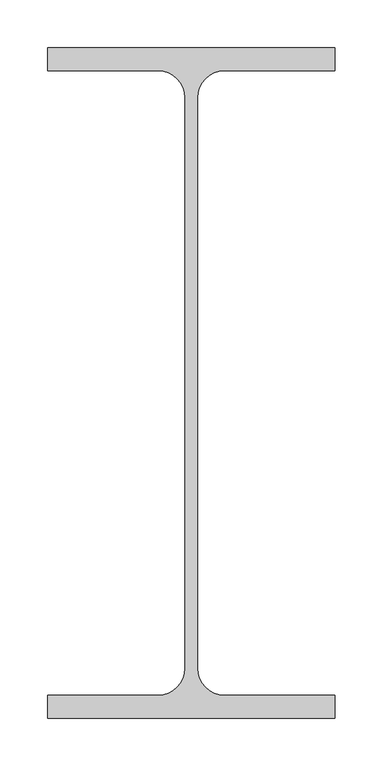
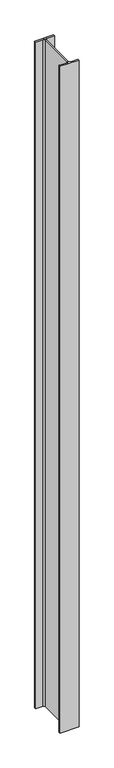
"""IFC4 building model written with IfcOpenShell, lengths in millimetres: column geometry, 0912_Steel Column_H_KSD3502 : H_SC_ASC_H-700x300x13x24."""

import ifcopenshell
import ifcopenshell.guid

model = None  # the IFC model being written
_history = None  # IfcOwnerHistory: only IFC2X3 demands one
_inside = {}  # id of a spatial element -> (the spatial element, [elements in it])
_under = {}  # id of a project, library or spatial element -> (it, [spatial elements below it])
_declared = {}  # id of a project -> (the project, [libraries it declares])
_typed = {}  # id of a type object -> (the type object, [elements of that type])
_made_of = {}  # id of a material, layer set ... -> (it, [elements and type objects made of it])


def new_model(schema):
    """Start an empty IFC model of exactly this schema.

    Asked for "IFC4X3", IfcOpenShell would pick the latest addendum, in which some entities
    have other attributes; the version numbers below select the first issue.
    IFC2X3 requires an IfcOwnerHistory on every rooted entity: one is made here for all.
    """
    global model, _history
    if schema == "IFC4X3":
        model = ifcopenshell.file(schema_version=(4, 3, 0, 0))
    else:
        model = ifcopenshell.file(schema=schema)
    _inside.clear()
    _under.clear()
    _declared.clear()
    _typed.clear()
    _made_of.clear()
    _history = None
    if model.schema == "IFC2X3":
        org = make("IfcOrganization", Name="unknown")
        user = make(
            "IfcPersonAndOrganization",
            ThePerson=make("IfcPerson", FamilyName="unknown"),
            TheOrganization=org,
        )
        app = make(
            "IfcApplication",
            ApplicationDeveloper=org,
            Version="unknown",
            ApplicationFullName="unknown",
            ApplicationIdentifier="unknown",
        )
        _history = make(
            "IfcOwnerHistory",
            OwningUser=user,
            OwningApplication=app,
            ChangeAction="ADDED",
            CreationDate=0,
        )
    return model


def make(cls, **values):
    """One entity of the class cls with the attributes given. An attribute that is None is left unset."""
    return model.create_entity(
        cls, **{name: value for name, value in values.items() if value is not None}
    )


def rooted(cls, **values):
    """An entity with a GlobalId (a new one), such as an element, a storey or a relation."""
    return make(cls, GlobalId=ifcopenshell.guid.new(), OwnerHistory=_history, **values)


def si_unit(unit_type, name, prefix=None):
    """IfcSIUnit, for example si_unit("LENGTHUNIT", "METRE", prefix="MILLI")."""
    return make("IfcSIUnit", UnitType=unit_type, Prefix=prefix, Name=name)


def assignment(units):
    """IfcUnitAssignment: the units of a project."""
    return None if units is None else make("IfcUnitAssignment", Units=units)


def point(xyz):
    """IfcCartesianPoint."""
    return None if xyz is None else make("IfcCartesianPoint", Coordinates=xyz)


def direction(xyz):
    """IfcDirection."""
    return None if xyz is None else make("IfcDirection", DirectionRatios=xyz)


def frame(location, z_axis=None, x_axis=None):
    """IfcAxis2Placement3D, a coordinate frame: its origin and axes. An axis left out is left unset."""
    return make(
        "IfcAxis2Placement3D",
        Location=point(location),
        Axis=direction(z_axis),
        RefDirection=direction(x_axis),
    )


def frame_2d(location, x_axis=None):
    """IfcAxis2Placement2D, a coordinate frame in the plane: its origin and x axis."""
    return make(
        "IfcAxis2Placement2D", Location=point(location), RefDirection=direction(x_axis)
    )


def origin():
    """The frame at (0, 0, 0) with its axes left unset."""
    return frame((0.0, 0.0, 0.0))


def origin_with_axes():
    """The frame at (0, 0, 0) with the z axis (0, 0, 1) and the x axis (1, 0, 0) written out."""
    return frame((0.0, 0.0, 0.0), z_axis=(0.0, 0.0, 1.0), x_axis=(1.0, 0.0, 0.0))


def place(relative_to, where):
    """IfcLocalPlacement: puts the frame where relative to a parent placement (None: the world)."""
    return make(
        "IfcLocalPlacement", PlacementRelTo=relative_to, RelativePlacement=where
    )


def context(
    kind, dimensions, precision=None, world=None, true_north=None, identifier=None
):
    """IfcGeometricRepresentationContext, for example the 3D "Model" context."""
    return make(
        "IfcGeometricRepresentationContext",
        ContextIdentifier=identifier,
        ContextType=kind,
        CoordinateSpaceDimension=dimensions,
        Precision=precision,
        WorldCoordinateSystem=world,
        TrueNorth=true_north,
    )


def project(units=None, contexts=None):
    """IfcProject with its units and contexts."""
    return rooted(
        "IfcProject",
        Name="project",
        RepresentationContexts=contexts,
        UnitsInContext=assignment(units),
    )


def spatial(cls, under=None, at=None, **own):
    """A site, building, storey or space (cls), placed at a placement, below another one or the project."""
    s = rooted(cls, ObjectPlacement=at, **own)
    if under is not None:
        _under.setdefault(under.id(), (under, []))[1].append(s)
    return s


def polyline(points):
    """IfcPolyline through the points."""
    return make("IfcPolyline", Points=[point(p) for p in points])


def circle_curve(where, radius):
    """IfcCircle in the frame where."""
    return make("IfcCircle", Position=where, Radius=radius)


def trimmed(basis, trim1, trim2, sense, master):
    """IfcTrimmedCurve: the piece of a basis curve between two trims."""
    return make(
        "IfcTrimmedCurve",
        BasisCurve=basis,
        Trim1=trim1,
        Trim2=trim2,
        SenseAgreement=sense,
        MasterRepresentation=master,
    )


def segment(curve, same_sense, transition):
    """IfcCompositeCurveSegment."""
    return make(
        "IfcCompositeCurveSegment",
        Transition=transition,
        SameSense=same_sense,
        ParentCurve=curve,
    )


def composite_curve(segments, self_intersect=None):
    """IfcCompositeCurve: segments joined end to end."""
    return make("IfcCompositeCurve", Segments=segments, SelfIntersect=self_intersect)


def outline(outer, holes=None, kind="AREA"):
    """IfcArbitraryClosedProfileDef: a profile drawn as a closed curve; with holes, ...WithVoids."""
    if holes is None:
        return make("IfcArbitraryClosedProfileDef", ProfileType=kind, OuterCurve=outer)
    return make(
        "IfcArbitraryProfileDefWithVoids",
        ProfileType=kind,
        OuterCurve=outer,
        InnerCurves=holes,
    )


def extrude(swept, where, along, depth):
    """IfcExtrudedAreaSolid: the profile swept, set in the frame where, extruded along a direction by depth."""
    return make(
        "IfcExtrudedAreaSolid",
        SweptArea=swept,
        Position=where,
        ExtrudedDirection=direction(along),
        Depth=depth,
    )


def shape(context_of_items, identifier, shape_type, items):
    """IfcShapeRepresentation: the items that make up one representation, for example the "Body"."""
    return make(
        "IfcShapeRepresentation",
        ContextOfItems=context_of_items,
        RepresentationIdentifier=identifier,
        RepresentationType=shape_type,
        Items=items,
    )


def source(mapping_origin, context_of_items, identifier, shape_type, items):
    """IfcRepresentationMap: a shape defined once, which mapped items show again and again."""
    return make(
        "IfcRepresentationMap",
        MappingOrigin=mapping_origin,
        MappedRepresentation=shape(context_of_items, identifier, shape_type, items),
    )


def transform(
    local_origin,
    x_axis=None,
    y_axis=None,
    z_axis=None,
    scale=None,
    scale2=None,
    scale3=None,
    uniform=True,
):
    """IfcCartesianTransformationOperator3D, or its non-uniform kind. x_axis, y_axis, z_axis: its Axis1, 2, 3."""
    if uniform:
        return make(
            "IfcCartesianTransformationOperator3D",
            Axis1=direction(x_axis),
            Axis2=direction(y_axis),
            LocalOrigin=point(local_origin),
            Scale=scale,
            Axis3=direction(z_axis),
        )
    return make(
        "IfcCartesianTransformationOperator3DnonUniform",
        Axis1=direction(x_axis),
        Axis2=direction(y_axis),
        LocalOrigin=point(local_origin),
        Scale=scale,
        Axis3=direction(z_axis),
        Scale2=scale2,
        Scale3=scale3,
    )


def mapped(mapping_source, mapping_target):
    """IfcMappedItem: shows the shape of a source again, moved by a transform."""
    return make(
        "IfcMappedItem", MappingSource=mapping_source, MappingTarget=mapping_target
    )


def made_of(thing, what):
    """Note that an element or type object is made of a material, layer set ...; save() writes the relation."""
    if what is not None:
        _made_of.setdefault(what.id(), (what, []))[1].append(thing)
    return thing


def element(
    cls,
    number,
    at=None,
    inside=None,
    cuts=None,
    type_object=None,
    material=None,
    context=None,
    identifier="Body",
    shape_type=None,
    held_by="IfcProductDefinitionShape",
    body=None,
    shapes=None,
    **own,
):
    """One element of the class cls, such as IfcWall. Its Tag is "e" and its number.

    at: its placement. inside: the storey or other place that contains it. cuts: it is an
    opening in that element (IfcRelVoidsElement). A single representation is given by context,
    identifier, shape_type and body (its items); several are given by shapes. held_by: the class
    of the entity that holds the representations. save() writes the other relations.
    """
    e = rooted(cls, Tag="e%d" % number, ObjectPlacement=at, **own)
    if body is not None:
        shapes = [shape(context, identifier, shape_type, body)]
    if shapes is not None:
        e.Representation = make(held_by, Representations=shapes)
    if inside is not None:
        _inside.setdefault(inside.id(), (inside, []))[1].append(e)
    if cuts is not None:
        rooted(
            "IfcRelVoidsElement", RelatingBuildingElement=cuts, RelatedOpeningElement=e
        )
    if type_object is not None:
        _typed.setdefault(type_object.id(), (type_object, []))[1].append(e)
    return made_of(e, material)


def aggregate(whole, parts):
    """IfcRelAggregates: a whole, such as a stair, and the parts it consists of."""
    return rooted("IfcRelAggregates", RelatingObject=whole, RelatedObjects=parts)


def save(model, path):
    """Write the relations noted so far, then the file.

    IfcRelAggregates (storeys below a building ...), IfcRelContainedInSpatialStructure (elements
    in a storey), IfcRelDefinesByType, IfcRelAssociatesMaterial and IfcRelDeclares: one each for
    every whole, place, type object, material and project.
    """
    for whole, parts in _under.values():
        aggregate(whole, parts)
    for where, things in _inside.values():
        rooted(
            "IfcRelContainedInSpatialStructure",
            RelatedElements=things,
            RelatingStructure=where,
        )
    for kind, things in _typed.values():
        rooted("IfcRelDefinesByType", RelatedObjects=things, RelatingType=kind)
    for what, things in _made_of.values():
        rooted("IfcRelAssociatesMaterial", RelatedObjects=things, RelatingMaterial=what)
    for by, libraries in _declared.values():
        rooted("IfcRelDeclares", RelatingContext=by, RelatedDefinitions=libraries)
    model.write(path)


def column_ca8bed04(model_context):
    return source(origin(), model_context, "Body", "SweptSolid", [
        extrude(outline(composite_curve([segment(polyline([(150.0, 350.0), (150.0, 326.0), (34.5, 326.0)]), True, "CONTINUOUS"), segment(trimmed(circle_curve(frame_2d((34.5, 298.0)), 28.0), [point((34.5, 326.0))], [point((6.5, 298.0))], True, "CARTESIAN"), True, "CONTINUOUS"), segment(polyline([(6.5, 298.0), (6.5, -298.0)]), True, "CONTINUOUS"), segment(trimmed(circle_curve(frame_2d((34.5, -298.0)), 28.0), [point((6.5, -298.0))], [point((34.5, -326.0))], True, "CARTESIAN"), True, "CONTINUOUS"), segment(polyline([(34.5, -326.0), (150.0, -326.0), (150.0, -350.0), (-150.0, -350.0), (-150.0, -326.0), (-34.5, -326.0)]), True, "CONTINUOUS"), segment(trimmed(circle_curve(frame_2d((-34.5, -298.0)), 28.0), [point((-34.5, -326.0))], [point((-6.5, -298.0))], True, "CARTESIAN"), True, "CONTINUOUS"), segment(polyline([(-6.5, -298.0), (-6.5, 298.0)]), True, "CONTINUOUS"), segment(trimmed(circle_curve(frame_2d((-34.5, 298.0)), 28.0), [point((-6.5, 298.0))], [point((-34.5, 326.0))], True, "CARTESIAN"), True, "CONTINUOUS"), segment(polyline([(-34.5, 326.0), (-150.0, 326.0), (-150.0, 350.0), (150.0, 350.0)]), True, "CONTINUOUS")], self_intersect=False)), origin_with_axes(), (0.0, 0.0, 1.0), 11224.0),
    ])


if __name__ == "__main__":
    model = new_model("IFC4")
    model_context = context("Model", 3, world=origin())
    ifc_project = project(units=[si_unit("LENGTHUNIT", "METRE", prefix="MILLI")], contexts=[model_context])
    site = spatial("IfcSite", under=ifc_project)
    building = spatial("IfcBuilding", under=site)
    placement = place(None, origin())
    column_shape = column_ca8bed04(model_context)
    element("IfcColumn", 1, ObjectType="0912_Steel Column_H_KSD3502 : H_SC_ASC_H-700x300x13x24", at=placement, inside=building, context=model_context, shape_type="MappedRepresentation", body=[
        mapped(column_shape, transform((0.0, 0.0, 0.0), x_axis=(1.0, 0.0, 0.0), y_axis=(0.0, 1.0, 0.0), z_axis=(0.0, 0.0, 1.0))),
    ])
    save(model, "model.ifc")

# Revit data of these elements
# Type "0912_Steel Column_H_KSD3502 : H_SC_ASC_H-700x300x13x24"
#   H_WM Code_1 = "S01AA002-00001 | Main Steel Structure Fabrication Work | Shelter/Building | Medium Steel - Standard (90KG/M>Weight≥30KG/M) | Material: (   )"
#   H_WM Code_2 = "S03AA028-00001 | Main Steel Structure Erection Work | Shelter/Building | Medium Steel (90KG/M>Weight≥30KG/M) | Material: (   )"
#   H_WM Code_3 = "S01AA010-00001 | Main Steel Structure Fabrication Work | Shelter/Building | Steel Painting/Coating | for Non-Fireproofed Steel Surface, Surface Preparation, Primer, Second & Final Coat | Material: (   )"
#   H_Q'ty Cal Type Tag = "SC-Q2"
#   Width = 30.0 cm
#   Web Thickness = 1.3 cm
#   Web Fillet = 2.8 cm
#   Warping Constant = 12338400.0 cm⁶
#   Torsional Moment of Inertia = 325.986 cm⁴
#   Section Area = 235.5 cm²
#   Plastic Modulus weak axis = 1120.0 cm³
#   Plastic Modulus strong axis = 6460.0 cm³
#   Perimeter = 2.53 m²/m
#   Nominal Weight = 185.00 kgf/m
#   Moment of Inertia weak axis = 10800.00 cm⁴
#   Moment of Inertia strong axis = 201000.00 cm⁴
#   Height = 70.0 cm
#   Flange Thickness = 2.4 cm
#   Elastic Modulus weak axis = 722.0 cm³
#   Elastic Modulus strong axis = 5760.0 cm³
#   Centroid Vertical = 35.0 cm
#   Centroid Horizontal = 15.0 cm
#   Structural Material [instance default] = Steel, 45-345
#   Section Name Key = ""
#   Bolt Spacing = 0
#   Assembly Code = ""
# Element 1 (IfcColumn, "0912_Steel Column_H_KSD3502 : H_SC_ASC_H-700x300x13x24")
#   Structural Material = A03AD029-00008_Anchor Bolt (Installation only)_M36
#   Materials on its faces: "A03AD029-00008_Anchor Bolt (Installation only)_M36"
# Materials
#   "Steel, 45-345": class "Metal", colour RGB 189 187 185, transparency 0, Description = "Steel 345 MPa", Cost = 0
#   "A03AD029-00008_Anchor Bolt (Installation only)_M36": class "Unassigned", colour RGB 84 83 81, transparency 0, Cost = 0
